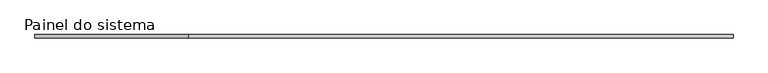
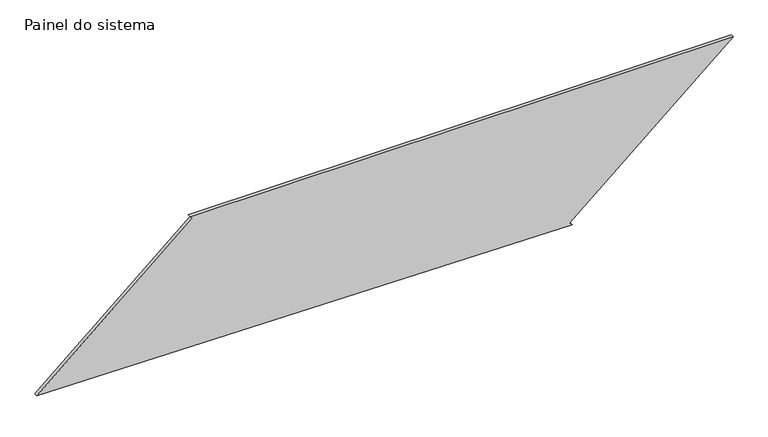
"""IFC4 building model written with IfcOpenShell, lengths in millimetres: plate geometry, Painel do sistema : Envidraçado."""

import ifcopenshell
import ifcopenshell.guid

model = None  # the IFC model being written
_history = None  # IfcOwnerHistory: only IFC2X3 demands one
_inside = {}  # id of a spatial element -> (the spatial element, [elements in it])
_under = {}  # id of a project, library or spatial element -> (it, [spatial elements below it])
_declared = {}  # id of a project -> (the project, [libraries it declares])
_typed = {}  # id of a type object -> (the type object, [elements of that type])
_made_of = {}  # id of a material, layer set ... -> (it, [elements and type objects made of it])


def new_model(schema):
    """Start an empty IFC model of exactly this schema.

    Asked for "IFC4X3", IfcOpenShell would pick the latest addendum, in which some entities
    have other attributes; the version numbers below select the first issue.
    IFC2X3 requires an IfcOwnerHistory on every rooted entity: one is made here for all.
    """
    global model, _history
    if schema == "IFC4X3":
        model = ifcopenshell.file(schema_version=(4, 3, 0, 0))
    else:
        model = ifcopenshell.file(schema=schema)
    _inside.clear()
    _under.clear()
    _declared.clear()
    _typed.clear()
    _made_of.clear()
    _history = None
    if model.schema == "IFC2X3":
        org = make("IfcOrganization", Name="unknown")
        user = make(
            "IfcPersonAndOrganization",
            ThePerson=make("IfcPerson", FamilyName="unknown"),
            TheOrganization=org,
        )
        app = make(
            "IfcApplication",
            ApplicationDeveloper=org,
            Version="unknown",
            ApplicationFullName="unknown",
            ApplicationIdentifier="unknown",
        )
        _history = make(
            "IfcOwnerHistory",
            OwningUser=user,
            OwningApplication=app,
            ChangeAction="ADDED",
            CreationDate=0,
        )
    return model


def make(cls, **values):
    """One entity of the class cls with the attributes given. An attribute that is None is left unset."""
    return model.create_entity(
        cls, **{name: value for name, value in values.items() if value is not None}
    )


def rooted(cls, **values):
    """An entity with a GlobalId (a new one), such as an element, a storey or a relation."""
    return make(cls, GlobalId=ifcopenshell.guid.new(), OwnerHistory=_history, **values)


def si_unit(unit_type, name, prefix=None):
    """IfcSIUnit, for example si_unit("LENGTHUNIT", "METRE", prefix="MILLI")."""
    return make("IfcSIUnit", UnitType=unit_type, Prefix=prefix, Name=name)


def assignment(units):
    """IfcUnitAssignment: the units of a project."""
    return None if units is None else make("IfcUnitAssignment", Units=units)


def point(xyz):
    """IfcCartesianPoint."""
    return None if xyz is None else make("IfcCartesianPoint", Coordinates=xyz)


def direction(xyz):
    """IfcDirection."""
    return None if xyz is None else make("IfcDirection", DirectionRatios=xyz)


def frame(location, z_axis=None, x_axis=None):
    """IfcAxis2Placement3D, a coordinate frame: its origin and axes. An axis left out is left unset."""
    return make(
        "IfcAxis2Placement3D",
        Location=point(location),
        Axis=direction(z_axis),
        RefDirection=direction(x_axis),
    )


def origin():
    """The frame at (0, 0, 0) with its axes left unset."""
    return frame((0.0, 0.0, 0.0))


def place(relative_to, where):
    """IfcLocalPlacement: puts the frame where relative to a parent placement (None: the world)."""
    return make(
        "IfcLocalPlacement", PlacementRelTo=relative_to, RelativePlacement=where
    )


def context(
    kind, dimensions, precision=None, world=None, true_north=None, identifier=None
):
    """IfcGeometricRepresentationContext, for example the 3D "Model" context."""
    return make(
        "IfcGeometricRepresentationContext",
        ContextIdentifier=identifier,
        ContextType=kind,
        CoordinateSpaceDimension=dimensions,
        Precision=precision,
        WorldCoordinateSystem=world,
        TrueNorth=true_north,
    )


def project(units=None, contexts=None):
    """IfcProject with its units and contexts."""
    return rooted(
        "IfcProject",
        Name="project",
        RepresentationContexts=contexts,
        UnitsInContext=assignment(units),
    )


def spatial(cls, under=None, at=None, **own):
    """A site, building, storey or space (cls), placed at a placement, below another one or the project."""
    s = rooted(cls, ObjectPlacement=at, **own)
    if under is not None:
        _under.setdefault(under.id(), (under, []))[1].append(s)
    return s


def polyline(points):
    """IfcPolyline through the points."""
    return make("IfcPolyline", Points=[point(p) for p in points])


def outline(outer, holes=None, kind="AREA"):
    """IfcArbitraryClosedProfileDef: a profile drawn as a closed curve; with holes, ...WithVoids."""
    if holes is None:
        return make("IfcArbitraryClosedProfileDef", ProfileType=kind, OuterCurve=outer)
    return make(
        "IfcArbitraryProfileDefWithVoids",
        ProfileType=kind,
        OuterCurve=outer,
        InnerCurves=holes,
    )


def extrude(swept, where, along, depth):
    """IfcExtrudedAreaSolid: the profile swept, set in the frame where, extruded along a direction by depth."""
    return make(
        "IfcExtrudedAreaSolid",
        SweptArea=swept,
        Position=where,
        ExtrudedDirection=direction(along),
        Depth=depth,
    )


def shape(context_of_items, identifier, shape_type, items):
    """IfcShapeRepresentation: the items that make up one representation, for example the "Body"."""
    return make(
        "IfcShapeRepresentation",
        ContextOfItems=context_of_items,
        RepresentationIdentifier=identifier,
        RepresentationType=shape_type,
        Items=items,
    )


def source(mapping_origin, context_of_items, identifier, shape_type, items):
    """IfcRepresentationMap: a shape defined once, which mapped items show again and again."""
    return make(
        "IfcRepresentationMap",
        MappingOrigin=mapping_origin,
        MappedRepresentation=shape(context_of_items, identifier, shape_type, items),
    )


def transform(
    local_origin,
    x_axis=None,
    y_axis=None,
    z_axis=None,
    scale=None,
    scale2=None,
    scale3=None,
    uniform=True,
):
    """IfcCartesianTransformationOperator3D, or its non-uniform kind. x_axis, y_axis, z_axis: its Axis1, 2, 3."""
    if uniform:
        return make(
            "IfcCartesianTransformationOperator3D",
            Axis1=direction(x_axis),
            Axis2=direction(y_axis),
            LocalOrigin=point(local_origin),
            Scale=scale,
            Axis3=direction(z_axis),
        )
    return make(
        "IfcCartesianTransformationOperator3DnonUniform",
        Axis1=direction(x_axis),
        Axis2=direction(y_axis),
        LocalOrigin=point(local_origin),
        Scale=scale,
        Axis3=direction(z_axis),
        Scale2=scale2,
        Scale3=scale3,
    )


def mapped(mapping_source, mapping_target):
    """IfcMappedItem: shows the shape of a source again, moved by a transform."""
    return make(
        "IfcMappedItem", MappingSource=mapping_source, MappingTarget=mapping_target
    )


def made_of(thing, what):
    """Note that an element or type object is made of a material, layer set ...; save() writes the relation."""
    if what is not None:
        _made_of.setdefault(what.id(), (what, []))[1].append(thing)
    return thing


def element(
    cls,
    number,
    at=None,
    inside=None,
    cuts=None,
    type_object=None,
    material=None,
    context=None,
    identifier="Body",
    shape_type=None,
    held_by="IfcProductDefinitionShape",
    body=None,
    shapes=None,
    **own,
):
    """One element of the class cls, such as IfcWall. Its Tag is "e" and its number.

    at: its placement. inside: the storey or other place that contains it. cuts: it is an
    opening in that element (IfcRelVoidsElement). A single representation is given by context,
    identifier, shape_type and body (its items); several are given by shapes. held_by: the class
    of the entity that holds the representations. save() writes the other relations.
    """
    e = rooted(cls, Tag="e%d" % number, ObjectPlacement=at, **own)
    if body is not None:
        shapes = [shape(context, identifier, shape_type, body)]
    if shapes is not None:
        e.Representation = make(held_by, Representations=shapes)
    if inside is not None:
        _inside.setdefault(inside.id(), (inside, []))[1].append(e)
    if cuts is not None:
        rooted(
            "IfcRelVoidsElement", RelatingBuildingElement=cuts, RelatedOpeningElement=e
        )
    if type_object is not None:
        _typed.setdefault(type_object.id(), (type_object, []))[1].append(e)
    return made_of(e, material)


def aggregate(whole, parts):
    """IfcRelAggregates: a whole, such as a stair, and the parts it consists of."""
    return rooted("IfcRelAggregates", RelatingObject=whole, RelatedObjects=parts)


def save(model, path):
    """Write the relations noted so far, then the file.

    IfcRelAggregates (storeys below a building ...), IfcRelContainedInSpatialStructure (elements
    in a storey), IfcRelDefinesByType, IfcRelAssociatesMaterial and IfcRelDeclares: one each for
    every whole, place, type object, material and project.
    """
    for whole, parts in _under.values():
        aggregate(whole, parts)
    for where, things in _inside.values():
        rooted(
            "IfcRelContainedInSpatialStructure",
            RelatedElements=things,
            RelatingStructure=where,
        )
    for kind, things in _typed.values():
        rooted("IfcRelDefinesByType", RelatedObjects=things, RelatingType=kind)
    for what, things in _made_of.values():
        rooted("IfcRelAssociatesMaterial", RelatedObjects=things, RelatingMaterial=what)
    for by, libraries in _declared.values():
        rooted("IfcRelDeclares", RelatingContext=by, RelatedDefinitions=libraries)
    model.write(path)


def painel_do_sistema_47bf2ed3(model_context):
    return source(origin(), model_context, "Body", "SweptSolid", [
        extrude(outline(polyline([(0.0, 1351.6711416), (19.0100862, 1335.4348667), (1026.5429997, 2515.0950787), (1026.5429997, -1407.6472841), (1007.5329135, -1391.4110092), (47.8085175, -2515.0950787), (0.0, 1351.6711416)])), frame((0.0, 24.5, 0.0), z_axis=(0.0, 1.0, 0.0), x_axis=(0.0, 0.0, 1.0)), (0.0, 0.0, 1.0), 25.0),
    ])


if __name__ == "__main__":
    model = new_model("IFC4")
    model_context = context("Model", 3, world=origin())
    ifc_project = project(units=[si_unit("LENGTHUNIT", "METRE", prefix="MILLI")], contexts=[model_context])
    site = spatial("IfcSite", under=ifc_project)
    building = spatial("IfcBuilding", under=site)
    placement = place(None, origin())
    painel_do_sistema_shape = painel_do_sistema_47bf2ed3(model_context)
    element("IfcPlate", 1, ObjectType="Painel do sistema : Envidraçado", at=placement, inside=building, context=model_context, shape_type="MappedRepresentation", body=[
        mapped(painel_do_sistema_shape, transform((0.0, 0.0, 0.0), x_axis=(1.0, 0.0, 0.0), y_axis=(0.0, 1.0, 0.0), z_axis=(0.0, 0.0, 1.0))),
    ])
    save(model, "model.ifc")

# Revit data of these elements
# Type "Painel do sistema : Envidraçado"
#   Construction Type Id = "GSP4R"
#   Analytic Construction = "Vidraça única Pilkington 1/8 pol"
#   Visual Light Transmittance = 0.9
#   Solar Heat Gain Coefficient = 0.86
#   Heat Transfer Coefficient (U) = 6.7069 W/(m²·K)
# Element 1 (IfcPlate, "Painel do sistema : Envidraçado")
#   Materials on its faces: "Vidro"
# Materials
#   "Vidro": class "Vidro", colour RGB 0 128 192, transparency 0.9, Description = "Vidro de sílica", Cost = 0
